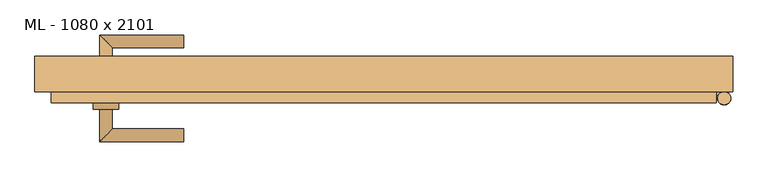
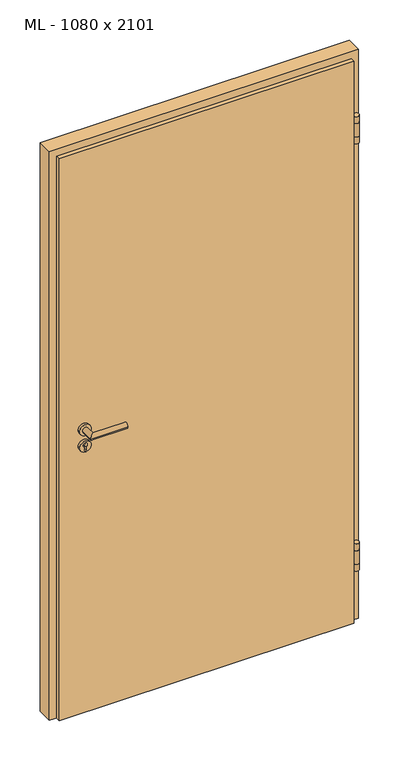
"""IFC4 building model written with IfcOpenShell, lengths in millimetres: door geometry, TU DF 1 - Pfostenstock Falztüre : ML - 1080 x 2101."""

from ifc_helpers import new_model, si_unit, point, frame, frame_2d, origin, place, context, project, spatial, polyline, circle_curve, ellipse_curve, trimmed, segment, composite_curve, outline, extrude, faceted_brep, source, transform, mapped, element, save
from ifc_brep_helpers import plane_surface, cylinder_surface, advanced_brep


def ml_1080_x_2101_9ecaf8c8(model_context):
    return source(origin(), model_context, "Body", "SolidModel", [
        faceted_brep([(515.0, -44.5, 0.0), (-515.0, -44.5, 0.0), (-515.0, -27.5, 0.0), (-500.0, -27.5, 0.0), (-500.0, 0.5, 0.0), (500.0, 0.5, 0.0), (500.0, -27.5, 0.0), (515.0, -27.5, 0.0), (515.0, -44.5, 2075.0), (-515.0, -44.5, 2075.0), (-515.0, -27.5, 2075.0), (-500.0, -27.5, 2060.0), (515.0, -27.5, 2075.0), (500.0, -27.5, 2060.0), (-500.0, 0.5, 2060.0), (500.0, 0.5, 2060.0)], [[[0, 1, 2, 3, 4, 5, 6, 7]], [[8, 9, 1, 0]], [[1, 9, 10, 2]], [[11, 3, 2, 10, 12, 7, 6, 13]], [[3, 11, 14, 4]], [[5, 4, 14, 15]], [[13, 6, 5, 15]], [[8, 0, 7, 12]], [[9, 8, 12, 10]], [[11, 13, 15, 14]]]),
        extrude(outline(composite_curve([segment(trimmed(circle_curve(frame_2d((527.0, -37.5)), 10.0), [point((517.0, -37.5))], [point((537.0, -37.5))], False, "CARTESIAN"), True, "CONTINUOUS"), segment(trimmed(circle_curve(frame_2d((527.0, -37.5)), 10.0), [point((537.0, -37.5))], [point((517.0, -37.5))], False, "CARTESIAN"), True, "CONTINUOUS")], self_intersect=False)), frame((0.0, 0.0, 1844.0), z_axis=(0.0, 0.0, 1.0), x_axis=(1.0, 0.0, 0.0)), (0.0, 0.0, 1.0), 25.0),
        extrude(outline(composite_curve([segment(trimmed(circle_curve(frame_2d((527.0, -37.5)), 10.0), [point((527.0, -27.5))], [point((518.339746, -32.5))], False, "CARTESIAN"), True, "CONTINUOUS"), segment(polyline([(518.339746, -32.5), (515.0, -32.5), (515.0, -27.5), (527.0, -27.5)]), True, "CONTINUOUS")], self_intersect=False)), frame((0.0, 0.0, 1794.0), z_axis=(0.0, 0.0, 1.0), x_axis=(1.0, 0.0, 0.0)), (0.0, 0.0, 1.0), 50.0),
        extrude(outline(composite_curve([segment(trimmed(circle_curve(frame_2d((527.0, -37.5)), 10.0), [point((517.0, -37.5))], [point((537.0, -37.5))], False, "CARTESIAN"), True, "CONTINUOUS"), segment(trimmed(circle_curve(frame_2d((527.0, -37.5)), 10.0), [point((537.0, -37.5))], [point((517.0, -37.5))], False, "CARTESIAN"), True, "CONTINUOUS")], self_intersect=False)), frame((0.0, 0.0, 1769.0), z_axis=(0.0, 0.0, 1.0), x_axis=(1.0, 0.0, 0.0)), (0.0, 0.0, 1.0), 25.0),
        extrude(outline(composite_curve([segment(trimmed(circle_curve(frame_2d((527.0, -37.5)), 10.0), [point((517.0, -37.5))], [point((537.0, -37.5))], False, "CARTESIAN"), True, "CONTINUOUS"), segment(trimmed(circle_curve(frame_2d((527.0, -37.5)), 10.0), [point((537.0, -37.5))], [point((517.0, -37.5))], False, "CARTESIAN"), True, "CONTINUOUS")], self_intersect=False)), frame((0.0, 0.0, 266.0), z_axis=(0.0, 0.0, 1.0), x_axis=(1.0, 0.0, 0.0)), (0.0, 0.0, 1.0), 25.0),
        extrude(outline(composite_curve([segment(trimmed(circle_curve(frame_2d((527.0, -37.5)), 10.0), [point((527.0, -27.5))], [point((518.339746, -32.5))], False, "CARTESIAN"), True, "CONTINUOUS"), segment(polyline([(518.339746, -32.5), (515.0, -32.5), (515.0, -27.5), (527.0, -27.5)]), True, "CONTINUOUS")], self_intersect=False)), frame((0.0, 0.0, 216.0), z_axis=(0.0, 0.0, 1.0), x_axis=(1.0, 0.0, 0.0)), (0.0, 0.0, 1.0), 50.0),
        extrude(outline(composite_curve([segment(trimmed(circle_curve(frame_2d((527.0, -37.5)), 10.0), [point((517.0, -37.5))], [point((537.0, -37.5))], False, "CARTESIAN"), True, "CONTINUOUS"), segment(trimmed(circle_curve(frame_2d((527.0, -37.5)), 10.0), [point((537.0, -37.5))], [point((517.0, -37.5))], False, "CARTESIAN"), True, "CONTINUOUS")], self_intersect=False)), frame((0.0, 0.0, 191.0), z_axis=(0.0, 0.0, 1.0), x_axis=(1.0, 0.0, 0.0)), (0.0, 0.0, 1.0), 25.0),
        advanced_brep(
        [(-420.0, -54.5, 1050.0), (-440.0, -54.5, 1050.0), (-440.0, -104.5, 1050.0), (-420.0, -84.5, 1050.0), (-310.0, -84.5, 1050.0), (-310.0, -104.5, 1050.0)],
        [
            (0, 1, circle_curve(frame((-430.0, -54.5, 1050.0), z_axis=(0.0, 1.0, 0.0), x_axis=(-1.0, 0.0, 0.0)), 10.0)),
            (1, 0, circle_curve(frame((-430.0, -54.5, 1050.0), z_axis=(0.0, 1.0, 0.0), x_axis=(-1.0, 0.0, 0.0)), 10.0)),
            (1, 2),
            (2, 3, ellipse_curve(frame((-430.0, -94.5, 1050.0), z_axis=(-0.7071067811865531, 0.7071067811865419, 0.0), x_axis=(0.707106781186542, 0.707106781186553, 0.0)), 14.1421356, 10.0)),
            (3, 0),
            (3, 2, ellipse_curve(frame((-430.0, -94.5, 1050.0), z_axis=(-0.7071067811865531, 0.7071067811865419, 0.0), x_axis=(0.707106781186542, 0.707106781186553, 0.0)), 14.1421356, 10.0)),
            (4, 5, circle_curve(frame((-310.0, -94.5, 1050.0), z_axis=(1.0, 0.0, 0.0), x_axis=(0.0, -1.0, 0.0)), 10.0)),
            (5, 4, circle_curve(frame((-310.0, -94.5, 1050.0), z_axis=(1.0, 0.0, 0.0), x_axis=(0.0, -1.0, 0.0)), 10.0)),
            (2, 5),
            (4, 3),
        ],
        [
            plane_surface(frame((-430.0, -54.5, 1050.0), z_axis=(0.0, 1.0, 0.0), x_axis=(0.0, 0.0, 1.0))),
            cylinder_surface(frame((-430.0, -54.5, 1050.0), z_axis=(0.0, 1.0, 0.0), x_axis=(-1.0, 0.0, 0.0)), 10.0),
            plane_surface(frame((-310.0, -94.5, 1050.0), z_axis=(1.0, 0.0, 0.0), x_axis=(0.0, 0.0, 1.0))),
            cylinder_surface(frame((-430.0, -94.5, 1050.0), z_axis=(-1.0, 0.0, 0.0), x_axis=(0.0, -1.0, 0.0)), 10.0),
        ],
        [
            (0, [[1, 2]]),
            (1, [[3, 4, 5, -2]]),
            (1, [[-5, 6, -3, -1]]),
            (2, [[7, 8]]),
            (3, [[9, -7, 10, -4]]),
            (3, [[-10, -8, -9, -6]]),
        ],
    ),
        extrude(outline(composite_curve([segment(trimmed(circle_curve(frame_2d((990.0, -430.0)), 20.0), [point((990.0, -450.0))], [point((990.0, -410.0))], False, "CARTESIAN"), True, "CONTINUOUS"), segment(trimmed(circle_curve(frame_2d((990.0, -430.0)), 20.0), [point((990.0, -410.0))], [point((990.0, -450.0))], False, "CARTESIAN"), True, "CONTINUOUS")], self_intersect=False), holes=[composite_curve([segment(polyline([(976.4601385, -432.397268), (988.4749012, -432.397268)]), True, "CONTINUOUS"), segment(trimmed(circle_curve(frame_2d((995.0361633, -430.0)), 6.9854888), [point((988.4749012, -432.397268))], [point((988.4749012, -427.602732))], True, "CARTESIAN"), True, "CONTINUOUS"), segment(polyline([(988.4749012, -427.602732), (976.4601385, -427.602732)]), True, "CONTINUOUS"), segment(trimmed(circle_curve(frame_2d((976.4601385, -430.0)), 2.397268), [point((976.4601385, -427.602732))], [point((976.4601385, -432.397268))], True, "CARTESIAN"), True, "CONTINUOUS")], self_intersect=False)]), frame((0.0, -54.5, 0.0), z_axis=(0.0, 1.0, 0.0), x_axis=(0.0, 0.0, 1.0)), (0.0, 0.0, 1.0), 10.0),
        advanced_brep(
        [(-420.0, -54.5, 1050.0), (-440.0, -54.5, 1050.0), (-440.0, -104.5, 1050.0), (-420.0, -84.5, 1050.0), (-310.0, -84.5, 1050.0), (-310.0, -104.5, 1050.0)],
        [
            (0, 1, circle_curve(frame((-430.0, -54.5, 1050.0), z_axis=(0.0, 1.0, 0.0), x_axis=(-1.0, 0.0, 0.0)), 10.0)),
            (1, 0, circle_curve(frame((-430.0, -54.5, 1050.0), z_axis=(0.0, 1.0, 0.0), x_axis=(-1.0, 0.0, 0.0)), 10.0)),
            (1, 2),
            (2, 3, ellipse_curve(frame((-430.0, -94.5, 1050.0), z_axis=(-0.7071067811865537, 0.7071067811865414, 0.0), x_axis=(0.7071067811865414, 0.7071067811865536, 0.0)), 14.1421356, 10.0)),
            (3, 0),
            (3, 2, ellipse_curve(frame((-430.0, -94.5, 1050.0), z_axis=(-0.7071067811865537, 0.7071067811865414, 0.0), x_axis=(0.7071067811865414, 0.7071067811865536, 0.0)), 14.1421356, 10.0)),
            (4, 5, circle_curve(frame((-310.0, -94.5, 1050.0), z_axis=(1.0, 0.0, 0.0), x_axis=(0.0, -1.0, 0.0)), 10.0)),
            (5, 4, circle_curve(frame((-310.0, -94.5, 1050.0), z_axis=(1.0, 0.0, 0.0), x_axis=(0.0, -1.0, 0.0)), 10.0)),
            (2, 5),
            (4, 3),
        ],
        [
            plane_surface(frame((-430.0, -54.5, 1050.0), z_axis=(0.0, 1.0, 0.0), x_axis=(0.0, 0.0, 1.0))),
            cylinder_surface(frame((-430.0, -54.5, 1050.0), z_axis=(0.0, 1.0, 0.0), x_axis=(-1.0, 0.0, 0.0)), 10.0),
            plane_surface(frame((-310.0, -94.5, 1050.0), z_axis=(1.0, 0.0, 0.0), x_axis=(0.0, 0.0, 1.0))),
            cylinder_surface(frame((-430.0, -94.5, 1050.0), z_axis=(-1.0, 0.0, 0.0), x_axis=(0.0, -1.0, 0.0)), 10.0),
        ],
        [
            (0, [[1, 2]]),
            (1, [[3, 4, 5, -2]]),
            (1, [[-5, 6, -3, -1]]),
            (2, [[7, 8]]),
            (3, [[9, -7, 10, -4]]),
            (3, [[-10, -8, -9, -6]]),
        ],
    ),
        extrude(outline(composite_curve([segment(trimmed(circle_curve(frame_2d((1050.0, -430.0)), 20.0), [point((1050.0, -450.0))], [point((1050.0, -410.0))], False, "CARTESIAN"), True, "CONTINUOUS"), segment(trimmed(circle_curve(frame_2d((1050.0, -430.0)), 20.0), [point((1050.0, -410.0))], [point((1050.0, -450.0))], False, "CARTESIAN"), True, "CONTINUOUS")], self_intersect=False)), frame((0.0, -54.5, 0.0), z_axis=(0.0, 1.0, 0.0), x_axis=(0.0, 0.0, 1.0)), (0.0, 0.0, 1.0), 10.0),
        advanced_brep(
        [(-420.0, 10.5, 1050.0), (-440.0, 10.5, 1050.0), (-420.0, 40.5, 1050.0), (-440.0, 60.5, 1050.0), (-310.0, 40.5, 1050.0), (-310.0, 60.5, 1050.0)],
        [
            (0, 1, circle_curve(frame((-430.0, 10.5, 1050.0), z_axis=(0.0, -1.0, 0.0), x_axis=(-1.0, 0.0, 0.0)), 10.0)),
            (1, 0, circle_curve(frame((-430.0, 10.5, 1050.0), z_axis=(0.0, -1.0, 0.0), x_axis=(-1.0, 0.0, 0.0)), 10.0)),
            (0, 2),
            (2, 3, ellipse_curve(frame((-430.0, 50.5, 1050.0), z_axis=(-0.7071067811865486, -0.7071067811865464, 0.0), x_axis=(0.7071067811865464, -0.7071067811865488, 0.0)), 14.1421356, 10.0)),
            (3, 1),
            (3, 2, ellipse_curve(frame((-430.0, 50.5, 1050.0), z_axis=(-0.7071067811865486, -0.7071067811865464, 0.0), x_axis=(0.7071067811865464, -0.7071067811865488, 0.0)), 14.1421356, 10.0)),
            (4, 5, circle_curve(frame((-310.0, 50.5, 1050.0), z_axis=(1.0, 0.0, 0.0), x_axis=(0.0, 1.0, 0.0)), 10.0)),
            (5, 4, circle_curve(frame((-310.0, 50.5, 1050.0), z_axis=(1.0, 0.0, 0.0), x_axis=(0.0, 1.0, 0.0)), 10.0)),
            (2, 4),
            (5, 3),
        ],
        [
            plane_surface(frame((-430.0, 10.5, 1050.0), z_axis=(0.0, -1.0, 0.0), x_axis=(0.0, 0.0, 1.0))),
            cylinder_surface(frame((-430.0, 10.5, 1050.0), z_axis=(0.0, -1.0, 0.0), x_axis=(-1.0, 0.0, 0.0)), 10.0),
            plane_surface(frame((-310.0, 50.5, 1050.0), z_axis=(1.0, 0.0, 0.0), x_axis=(0.0, 0.0, 1.0))),
            cylinder_surface(frame((-430.0, 50.5, 1050.0), z_axis=(-1.0, 0.0, 0.0), x_axis=(0.0, 1.0, 0.0)), 10.0),
        ],
        [
            (0, [[1, 2]]),
            (1, [[-1, 3, 4, 5]]),
            (1, [[-2, -5, 6, -3]]),
            (2, [[7, 8]]),
            (3, [[-4, 9, -8, 10]]),
            (3, [[-6, -10, -7, -9]]),
        ],
    ),
        extrude(outline(composite_curve([segment(trimmed(circle_curve(frame_2d((990.0, -430.0)), 20.0), [point((990.0, -450.0))], [point((990.0, -410.0))], False, "CARTESIAN"), True, "CONTINUOUS"), segment(trimmed(circle_curve(frame_2d((990.0, -430.0)), 20.0), [point((990.0, -410.0))], [point((990.0, -450.0))], False, "CARTESIAN"), True, "CONTINUOUS")], self_intersect=False), holes=[composite_curve([segment(polyline([(976.4601385, -432.397268), (988.4749012, -432.397268)]), True, "CONTINUOUS"), segment(trimmed(circle_curve(frame_2d((995.0361633, -430.0)), 6.9854888), [point((988.4749012, -432.397268))], [point((988.4749012, -427.602732))], True, "CARTESIAN"), True, "CONTINUOUS"), segment(polyline([(988.4749012, -427.602732), (976.4601385, -427.602732)]), True, "CONTINUOUS"), segment(trimmed(circle_curve(frame_2d((976.4601385, -430.0)), 2.397268), [point((976.4601385, -427.602732))], [point((976.4601385, -432.397268))], True, "CARTESIAN"), True, "CONTINUOUS")], self_intersect=False)]), frame((0.0, 0.5, 0.0), z_axis=(0.0, 1.0, 0.0), x_axis=(0.0, 0.0, 1.0)), (0.0, 0.0, 1.0), 10.0),
        advanced_brep(
        [(-420.0, 10.5, 1050.0), (-440.0, 10.5, 1050.0), (-420.0, 40.5, 1050.0), (-440.0, 60.5, 1050.0), (-310.0, 40.5, 1050.0), (-310.0, 60.5, 1050.0)],
        [
            (0, 1, circle_curve(frame((-430.0, 10.5, 1050.0), z_axis=(0.0, -1.0, 0.0), x_axis=(-1.0, 0.0, 0.0)), 10.0)),
            (1, 0, circle_curve(frame((-430.0, 10.5, 1050.0), z_axis=(0.0, -1.0, 0.0), x_axis=(-1.0, 0.0, 0.0)), 10.0)),
            (0, 2),
            (2, 3, ellipse_curve(frame((-430.0, 50.5, 1050.0), z_axis=(-0.7071067811865491, -0.7071067811865459, 0.0), x_axis=(0.7071067811865458, -0.7071067811865492, 0.0)), 14.1421356, 10.0)),
            (3, 1),
            (3, 2, ellipse_curve(frame((-430.0, 50.5, 1050.0), z_axis=(-0.7071067811865491, -0.7071067811865459, 0.0), x_axis=(0.7071067811865458, -0.7071067811865492, 0.0)), 14.1421356, 10.0)),
            (4, 5, circle_curve(frame((-310.0, 50.5, 1050.0), z_axis=(1.0, 0.0, 0.0), x_axis=(0.0, 1.0, 0.0)), 10.0)),
            (5, 4, circle_curve(frame((-310.0, 50.5, 1050.0), z_axis=(1.0, 0.0, 0.0), x_axis=(0.0, 1.0, 0.0)), 10.0)),
            (2, 4),
            (5, 3),
        ],
        [
            plane_surface(frame((-430.0, 10.5, 1050.0), z_axis=(0.0, -1.0, 0.0), x_axis=(0.0, 0.0, 1.0))),
            cylinder_surface(frame((-430.0, 10.5, 1050.0), z_axis=(0.0, -1.0, 0.0), x_axis=(-1.0, 0.0, 0.0)), 10.0),
            plane_surface(frame((-310.0, 50.5, 1050.0), z_axis=(1.0, 0.0, 0.0), x_axis=(0.0, 0.0, 1.0))),
            cylinder_surface(frame((-430.0, 50.5, 1050.0), z_axis=(-1.0, 0.0, 0.0), x_axis=(0.0, 1.0, 0.0)), 10.0),
        ],
        [
            (0, [[1, 2]]),
            (1, [[-1, 3, 4, 5]]),
            (1, [[-2, -5, 6, -3]]),
            (2, [[7, 8]]),
            (3, [[-4, 9, -8, 10]]),
            (3, [[-6, -10, -7, -9]]),
        ],
    ),
        extrude(outline(composite_curve([segment(trimmed(circle_curve(frame_2d((1050.0, -430.0)), 20.0), [point((1050.0, -450.0))], [point((1050.0, -410.0))], False, "CARTESIAN"), True, "CONTINUOUS"), segment(trimmed(circle_curve(frame_2d((1050.0, -430.0)), 20.0), [point((1050.0, -410.0))], [point((1050.0, -450.0))], False, "CARTESIAN"), True, "CONTINUOUS")], self_intersect=False)), frame((0.0, 0.5, 0.0), z_axis=(0.0, 1.0, 0.0), x_axis=(0.0, 0.0, 1.0)), (0.0, 0.0, 1.0), 10.0),
        faceted_brep([(-500.0, -27.5, 0.0), (-540.0, -27.5, 0.0), (-540.0, 27.5, 0.0), (-485.0, 27.5, 0.0), (-485.0, 0.5, 0.0), (-500.0, 0.5, 0.0), (-500.0, 0.5, 2060.0), (-500.0, -27.5, 2060.0), (-485.0, 0.5, 2045.0), (485.0, 0.5, 2045.0), (485.0, 0.5, 0.0), (500.0, 0.5, 0.0), (500.0, 0.5, 2060.0), (-485.0, 27.5, 2045.0), (-540.0, 27.5, 2100.0), (540.0, 27.5, 2100.0), (540.0, 27.5, 0.0), (485.0, 27.5, 0.0), (485.0, 27.5, 2045.0), (-540.0, -27.5, 2100.0), (500.0, -27.5, 2060.0), (500.0, -27.5, 0.0), (540.0, -27.5, 0.0), (540.0, -27.5, 2100.0)], [[[0, 1, 2, 3, 4, 5]], [[5, 6, 7, 0]], [[4, 8, 9, 10, 11, 12, 6, 5]], [[3, 13, 8, 4]], [[2, 14, 15, 16, 17, 18, 13, 3]], [[1, 19, 14, 2]], [[0, 7, 20, 21, 22, 23, 19, 1]], [[23, 22, 16, 15]], [[21, 11, 10, 17, 16, 22]], [[12, 11, 21, 20]], [[18, 17, 10, 9]], [[19, 23, 15, 14]], [[13, 18, 9, 8]], [[6, 12, 20, 7]]]),
    ])


if __name__ == "__main__":
    model = new_model("IFC4")
    model_context = context("Model", 3, world=origin())
    ifc_project = project(units=[si_unit("LENGTHUNIT", "METRE", prefix="MILLI")], contexts=[model_context])
    site = spatial("IfcSite", under=ifc_project)
    building = spatial("IfcBuilding", under=site)
    placement = place(None, origin())
    ml_1080_x_2101_shape = ml_1080_x_2101_9ecaf8c8(model_context)
    element("IfcDoor", 1, ObjectType="TU DF 1 - Pfostenstock Falztüre : ML - 1080 x 2101", at=placement, inside=building, context=model_context, shape_type="MappedRepresentation", body=[
        mapped(ml_1080_x_2101_shape, transform((0.0, 0.0, 0.0), x_axis=(1.0, 0.0, 0.0), y_axis=(0.0, 1.0, 0.0), z_axis=(0.0, 0.0, 1.0))),
    ])
    save(model, "model.ifc")

# Revit data of these elements
# Type "TU DF 1 - Pfostenstock Falztüre : ML - 1080 x 2101"
#   Type IfcGUID = "32vBIxahr8bQdQw1D1hUMo"
#   Type Mark = "235"
#   Operation = "SINGLE_SWING_RIGHT"
#   URL = "http://www.autodesk.de/BIM"
#   Type Comments = "Pfostenstock Falztüre"
#   Form Tür = "rechteckig"
#   Description = "1-teilig"
#   Ausführung Zarge = "Blockzarge"
#   Anzahl Seitenteile = "0"
#   Anzahl Oberlichter = "0"
#   Anzahl Flügel = "einflügelig"
#   Anschlag- / Bewegungsart Tür = "Drehflügeltür"
#   Analytic Construction = "<Keine Auswahl>"
#   Winkel Öffnungsbogen [instance default] = 90.00°
#   Wandstärke Gesamt [instance default] = 0.300 m
#   Wandstärke [instance default] = 0.300 m
#   Wandaufbau Gegenbandseite [instance default] = 0.000 m
#   Wandaufbau Bandseite [instance default] = 0.000 m
#   Rough Height [instance default] = 2.280 m
#   Rough Width = 1.080 m
#   Randabstand Öffnungssymbol = 0.000 m
#   Rahmentiefe = 0.055 m
#   Rahmendicke = 0.055 m
#   Höhe ab FBOK = 2.100 m
#   Fußbodenaufbau [instance default] = 0.180 m
#   Height [instance default] = 2.100 m
#   Falztiefe = 0.028 m
#   Falzaufschlag = 0.017 m
#   Einbautiefe [instance default] = 0.080 m
#   Durchgangshöhe = 2.045 m
#   Durchgangsbreite = 0.970 m
#   Drückerhöhe = 1.050 m
#   Thickness = 0.045 m
#   Width = 1.080 m
#   B_Einbautiefe [instance default] = 0.1225 m
#   Angabe Maueröffnungsmaß Höhe = 2.100 m
#   Angabe Maueröffnungsmaß Breite = 1.080 m
#   Angabe Lichter Durchgang Höhe = 2.000 m
#   Angabe Lichter Durchgang Breite = 0.800 m
#   Zylinderrosette [instance default] = yes
#   Tür mit Anschlag [instance default] = no
#   Pfostenstock Wandmittig eingebaut [instance default] = yes
#   Kollisionskörper einschalten [instance default] = no
#   Knauf Innenseite [instance default] = no
#   Knauf Außenseite [instance default] = no
#   Höhe ab FBOK berechnen = yes
#   Größenberechnung über Maueröffnungsmaß = yes
#   Größenberechnung über Lichten Durchgang = no
#   Grundrissdarstellung Türsturz [instance default] = no
#   Drücker Bandseite [instance default] = yes
#   Drücker Gegenbandseite [instance default] = yes
#   Türblatt [instance default] = none
#   Sichtbeschläge [instance default] = none
#   Rahmen vertikal [instance default] = none
#   Rahmen horizontal [instance default] = none
#   Kollisionskörper [instance default] = none
#   Function = (empty or 0)
#   Wall Closure = (empty or 0)
#   Fire Rating = ""
# Element 1 (IfcDoor, "TU DF 1 - Pfostenstock Falztüre : ML - 1080 x 2101")
#   Wandstärke Gesamt = 0.120 m
#   Wandstärke = 0.120 m
#   Rough Height = 2.100 m
#   Fußbodenaufbau = 0.000 m
#   B_Einbautiefe = 0.0325 m
#   Türblatt = Holz
#   Materials on its faces: "Metall - Edelstahl gebürstet", "Lack - grau 80-80-80", "Holz"
# Materials
#   "Metall - Edelstahl gebürstet": class "Metall", colour RGB 203 203 203, transparency 0, Description = "Edelstahl gebürstet", Cost = 0
#   "Lack - grau 80-80-80": class "Farbe/Beschichtung", colour RGB 80 80 80, transparency 0, Description = "Lack - grau 80-80-80", Cost = 0
#   "Holz": class "Holz", colour RGB 218 191 173, transparency 0, Description = "Holz - C 20 Cl.1", Cost = 0
